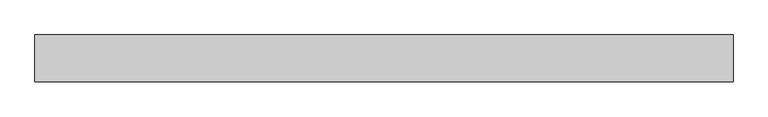
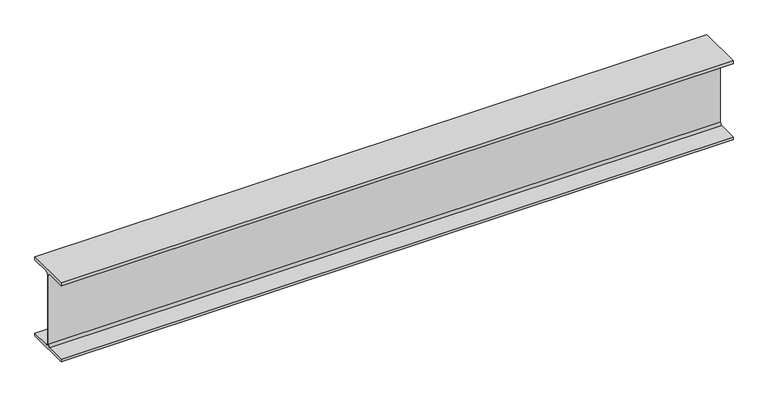
"""IFC4 building model written with IfcOpenShell, lengths in millimetres: beam geometry, Steel Beam_H-KSD3502 : H_SB_ASB_H-194x150x6x9."""

from ifc_helpers import new_model, si_unit, point, frame, frame_2d, origin, place, context, project, spatial, polyline, circle_curve, trimmed, segment, composite_curve, outline, extrude, source, transform, mapped, element, save


def beam_14fd6036(model_context):
    return source(origin(), model_context, "Body", "SweptSolid", [
        extrude(outline(composite_curve([segment(polyline([(-82.5, -141.5), (-11.9, -141.5)]), True, "CONTINUOUS"), segment(trimmed(circle_curve(frame_2d((-11.9, -132.6)), 8.9), [point((-11.9, -141.5))], [point((-3.0, -132.6))], True, "CARTESIAN"), True, "CONTINUOUS"), segment(polyline([(-3.0, -132.6), (-3.0, 132.6)]), True, "CONTINUOUS"), segment(trimmed(circle_curve(frame_2d((-11.9, 132.6)), 8.9), [point((-3.0, 132.6))], [point((-11.9, 141.5))], True, "CARTESIAN"), True, "CONTINUOUS"), segment(polyline([(-11.9, 141.5), (-82.5, 141.5), (-82.5, 151.7), (82.5, 151.7), (82.5, 141.5), (11.9, 141.5)]), True, "CONTINUOUS"), segment(trimmed(circle_curve(frame_2d((11.9, 132.6)), 8.9), [point((11.9, 141.5))], [point((3.0, 132.6))], True, "CARTESIAN"), True, "CONTINUOUS"), segment(polyline([(3.0, 132.6), (3.0, -132.6)]), True, "CONTINUOUS"), segment(trimmed(circle_curve(frame_2d((11.9, -132.6)), 8.9), [point((3.0, -132.6))], [point((11.9, -141.5))], True, "CARTESIAN"), True, "CONTINUOUS"), segment(polyline([(11.9, -141.5), (82.5, -141.5), (82.5, -151.7), (-82.5, -151.7), (-82.5, -141.5)]), True, "CONTINUOUS")], self_intersect=False)), frame((-1200.0, 0.0, 0.0), z_axis=(1.0, 0.0, 0.0), x_axis=(0.0, 1.0, 0.0)), (0.0, 0.0, 1.0), 2448.0465428),
    ])


if __name__ == "__main__":
    model = new_model("IFC4")
    model_context = context("Model", 3, world=origin())
    ifc_project = project(units=[si_unit("LENGTHUNIT", "METRE", prefix="MILLI")], contexts=[model_context])
    site = spatial("IfcSite", under=ifc_project)
    building = spatial("IfcBuilding", under=site)
    placement = place(None, origin())
    beam_shape = beam_14fd6036(model_context)
    element("IfcBeam", 1, ObjectType="Steel Beam_H-KSD3502 : H_SB_ASB_H-194x150x6x9", at=placement, inside=building, context=model_context, shape_type="MappedRepresentation", body=[
        mapped(beam_shape, transform((0.0, 0.0, 0.0), x_axis=(1.0, 0.0, 0.0), y_axis=(0.0, 1.0, 0.0), z_axis=(0.0, 0.0, 1.0))),
    ])
    save(model, "model.ifc")

# Revit data of these elements
# Type "Steel Beam_H-KSD3502 : H_SB_ASB_H-194x150x6x9"
#   Width = 15.0 cm
#   Web Thickness = 0.6 cm
#   Web Fillet = 1.3 cm
#   Warping Constant = 43316.0 cm⁶
#   Torsional Moment of Inertia = 8.622 cm⁴
#   Torsional Modulus = 1.0 cm³
#   Section Area = 39.01 cm²
#   Plastic Modulus weak axis = 104.0 cm³
#   Plastic Modulus strong axis = 309.0 cm³
#   Perimeter = 0.95 m²/m
#   Nominal Weight = 30.60 kgf/m
#   Moment of Inertia weak axis = 507.00 cm⁴
#   Moment of Inertia strong axis = 2690.00 cm⁴
#   Height = 19.4 cm
#   Flange Thickness = 0.9 cm
#   Elastic Modulus weak axis = 67.6 cm³
#   Elastic Modulus strong axis = 277.0 cm³
#   Centroid Vertical = 9.7 cm
#   Centroid Horizontal = 7.5 cm
#   Length [instance default] = 1.5240 m
#   Structural Material [instance default] = Steel, 45-345
#   Assembly Code = ""
# Element 1 (IfcBeam, "Steel Beam_H-KSD3502 : H_SB_ASB_H-194x150x6x9")
#   Structural Material = none
# Materials
#   "Steel, 45-345": class "Metal", colour RGB 189 187 185, transparency 0, Description = "Steel 345 MPa", Cost = 0
